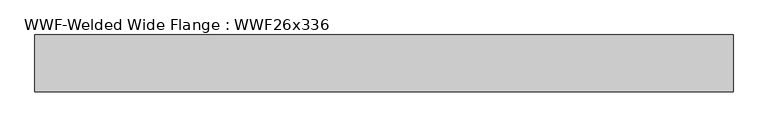
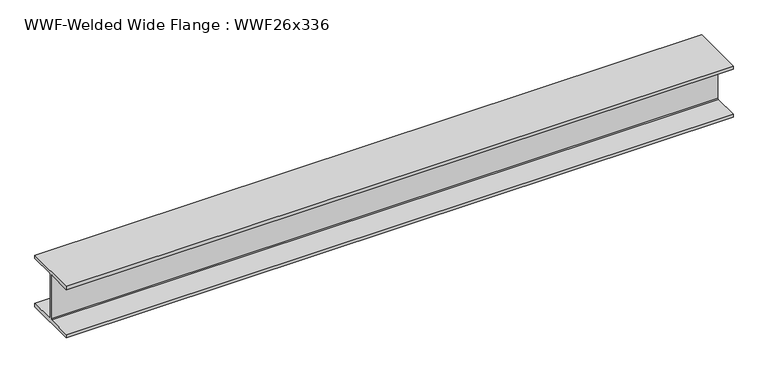
"""IFC4 building model written with IfcOpenShell, lengths in millimetres: beam geometry, WWF-Welded Wide Flange : WWF26x336."""

from ifc_helpers import new_model, si_unit, frame, origin, place, context, project, spatial, polyline, outline, extrude, source, transform, mapped, element, save


def wwf_welded_wide_flange_wwf26x336_896f099a(model_context):
    return source(origin(), model_context, "Body", "SweptSolid", [
        extrude(outline(polyline([(324.993, -284.988), (324.993, -324.993), (-324.993, -324.993), (-324.993, -284.988), (-20.6375, -284.988), (-9.9949, -274.3454), (-9.9949, 274.3454), (-20.6375, 284.988), (-324.993, 284.988), (-324.993, 324.993), (324.993, 324.993), (324.993, 284.988), (20.6375, 284.988), (9.9949, 274.3454), (9.9949, -274.3454), (20.6375, -284.988), (324.993, -284.988)])), frame((-3827.7582557, 0.0, 0.0), z_axis=(1.0, 0.0, 0.0), x_axis=(0.0, 1.0, 0.0)), (0.0, 0.0, 1.0), 7985.2347359),
    ])


if __name__ == "__main__":
    model = new_model("IFC4")
    model_context = context("Model", 3, world=origin())
    ifc_project = project(units=[si_unit("LENGTHUNIT", "METRE", prefix="MILLI")], contexts=[model_context])
    site = spatial("IfcSite", under=ifc_project)
    building = spatial("IfcBuilding", under=site)
    placement = place(None, origin())
    wwf_welded_wide_flange_wwf26x336_shape = wwf_welded_wide_flange_wwf26x336_896f099a(model_context)
    element("IfcBeam", 1, ObjectType="WWF-Welded Wide Flange : WWF26x336", at=placement, inside=building, context=model_context, shape_type="MappedRepresentation", body=[
        mapped(wwf_welded_wide_flange_wwf26x336_shape, transform((0.0, 0.0, 0.0), x_axis=(1.0, 0.0, 0.0), y_axis=(0.0, 1.0, 0.0), z_axis=(0.0, 0.0, 1.0))),
    ])
    save(model, "model.ifc")

# Revit data of these elements
# Type "WWF-Welded Wide Flange : WWF26x336"
#   Assembly Code = "B10"
#   Nominal d = "12"
#   W = 336
#   Length [instance default] = 1524 mm
#   bf = 649.986 mm
#   d = 649.986 mm
#   k = 20.638 mm
#   tf = 40.005 mm
#   tw = 19.99 mm
#   A = 0.0635483 m²
#   Structural Material [instance default] = Steel ASTM A572
# Element 1 (IfcBeam, "WWF-Welded Wide Flange : WWF26x336")
#   Structural Material = Metal - Steel 43-275
#   Materials on its faces: "Metal - Steel 43-275"
# Materials
#   "Steel ASTM A572": class "Metal", colour RGB 247 247 247, transparency 0, Description = "Structural steel, high strength low alloy, ASTM - A572 - 50", Cost = 0
#   "Metal - Steel 43-275": class "Metal", colour RGB 247 247 247, transparency 0, Cost = 0
